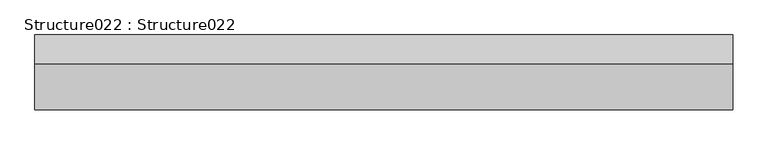
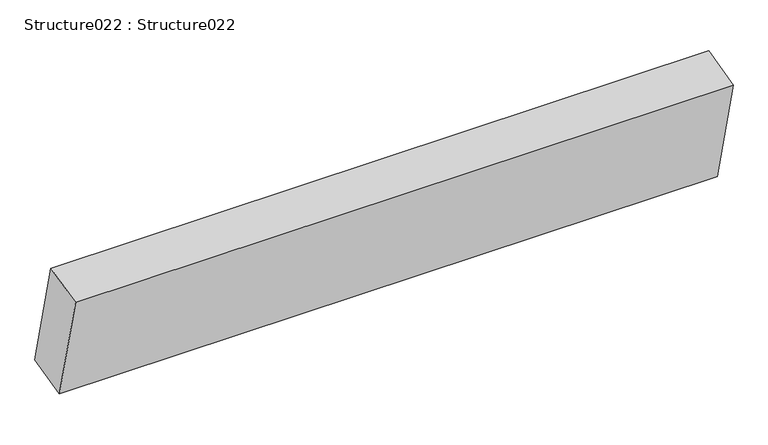
"""IFC4 building model written with IfcOpenShell, lengths in millimetres: proxy geometry, Structure022 : Structure022."""

from ifc_helpers import new_model, si_unit, frame, origin, place, context, project, spatial, polyline, outline, extrude, source, transform, mapped, element, save


def structure022_structure022_617f95eb(model_context):
    return source(origin(), model_context, "Body", "SweptSolid", [
        extrude(outline(polyline([(0.0, -133.35), (0.0, 0.0), (2000.0, 0.0), (2000.0, -133.35), (0.0, -133.35)])), frame((14383.0178845, -5447.9743192, 42379.6308633), z_axis=(0.0, -0.2379866304235585, 0.9712684303217317), x_axis=(-1.0, 0.0, 0.0)), (0.0, 0.0, 1.0), 355.6),
    ])


if __name__ == "__main__":
    model = new_model("IFC4")
    model_context = context("Model", 3, world=origin())
    ifc_project = project(units=[si_unit("LENGTHUNIT", "METRE", prefix="MILLI")], contexts=[model_context])
    site = spatial("IfcSite", under=ifc_project)
    building = spatial("IfcBuilding", under=site)
    placement = place(None, origin())
    structure022_structure022_shape = structure022_structure022_617f95eb(model_context)
    element("IfcBuildingElementProxy", 1, Name="Structure022 : Structure022", ObjectType="Structure022 : Structure022", at=placement, inside=building, context=model_context, shape_type="MappedRepresentation", body=[
        mapped(structure022_structure022_shape, transform((0.0, 0.0, 0.0), x_axis=(1.0, 0.0, 0.0), y_axis=(0.0, 1.0, 0.0), z_axis=(0.0, 0.0, 1.0))),
    ])
    save(model, "model.ifc")

# Revit data of these elements
# Type "Structure022 : Structure022"
#   NameOverride = "Structure022"
# Element 1 (IfcBuildingElementProxy, "Structure022 : Structure022")
#   Materials on its faces: "STRUCTURAL MEMBER (SEE STRUCTURAL DWGS)"
# Materials
#   "STRUCTURAL MEMBER (SEE STRUCTURAL DWGS)": class "Unassigned", colour RGB 176 134 95, transparency 0, Cost = 0
